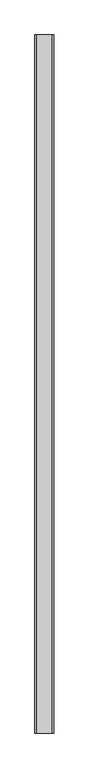
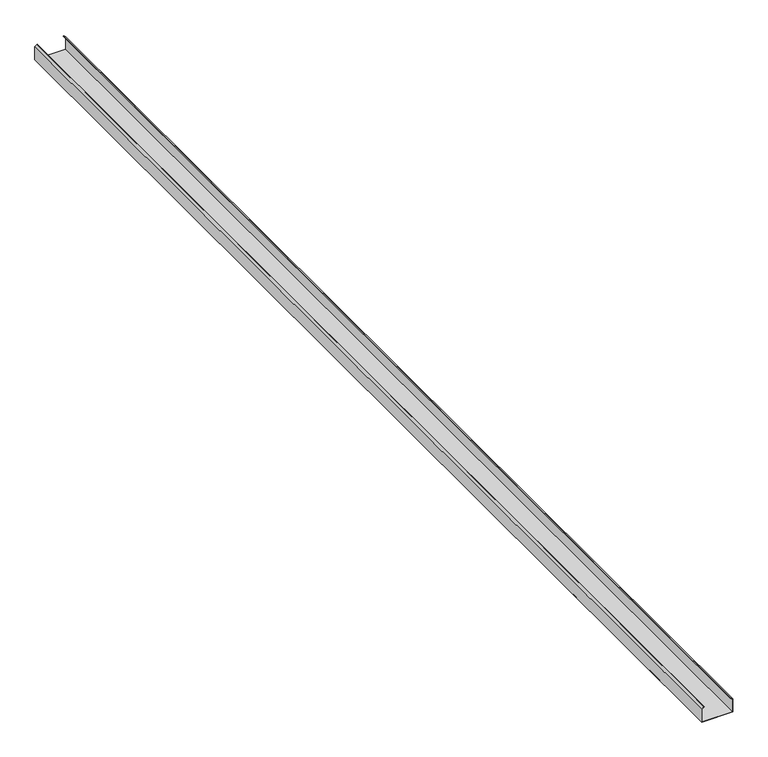
"""IFC4 building model written with IfcOpenShell, lengths in millimetres: proxy geometry, Generic Models 7:Generic Models 1:1:Generic Models 1:1 : Generic Models 7:Generic Models 1:337419:30 : Generic Models 7:Generic Models 1:1:Generic Models 1:1 : Generic Models 7:Generic Models 1:337419:306201."""

from ifc_helpers import new_model, si_unit, frame, origin, place, context, project, spatial, polyline, outline, extrude, source, transform, mapped, element, save


def generic_models_a6c114fe(model_context):
    return source(origin(), model_context, "Body", "SweptSolid", [
        extrude(outline(polyline([(2446.5359375, 667293.3117239), (2446.5359375, 667496.5117239), (2535.4359375, 667496.5117239), (2547.6810414, 667481.9185773), (2545.5528742, 667480.132833), (2534.1404765, 667493.7335989), (2449.3140625, 667493.7335989), (2449.3140625, 667296.0898489), (2534.1404765, 667296.0898489), (2545.5528742, 667309.6906149), (2547.6810414, 667307.9048706), (2535.4359375, 667293.3117239), (2446.5359375, 667293.3117239)])), frame((0.0, -507687.0163841, 0.0), z_axis=(0.0, 1.0, 0.0), x_axis=(0.0, 0.0, 1.0)), (0.0, 0.0, 1.0), 7569.2),
    ])


if __name__ == "__main__":
    model = new_model("IFC4")
    model_context = context("Model", 3, world=origin())
    ifc_project = project(units=[si_unit("LENGTHUNIT", "METRE", prefix="MILLI")], contexts=[model_context])
    site = spatial("IfcSite", under=ifc_project)
    building = spatial("IfcBuilding", under=site)
    placement = place(None, origin())
    generic_models_shape = generic_models_a6c114fe(model_context)
    element("IfcBuildingElementProxy", 1, Name="Generic Models 7:Generic Models 1:1:Generic Models 1:1 : Generic Models 7:Generic Models 1:337419:30 : Generic Models 7:Generic Models 1:1:Generic Models 1:1 : Generic Models 7:Generic Models 1:337419:306201", ObjectType="Generic Models 7:Generic Models 1:1:Generic Models 1:1 : Generic Models 7:Generic Models 1:337419:30 : Generic Models 7:Generic Models 1:1:Generic Models 1:1 : Generic Models 7:Generic Models 1:337419:306201", at=placement, inside=building, context=model_context, shape_type="MappedRepresentation", body=[
        mapped(generic_models_shape, transform((0.0, 0.0, 0.0), x_axis=(1.0, 0.0, 0.0), y_axis=(0.0, 1.0, 0.0), z_axis=(0.0, 0.0, 1.0))),
    ])
    save(model, "model.ifc")

# Revit data of these elements
# Type "Generic Models 7:Generic Models 1:1:Generic Models 1:1 : Generic Models 7:Generic Models 1:337419:30 : Generic Models 7:Generic Models 1:1:Generic Models 1:1 : Generic Models 7:Generic Models 1:337419:306201"
#   NameOverride = "Generic Models 7:Generic Models 1:1:Generic Models 1:1 : Generic Models 7:Generic Models 1:337419:306201"
#   ObjectTypeOverride = "Generic Models 1:1 : Generic Models 7:Generic Models 1:337419"
#   Reference = "Generic Models 1"
#   Tag = "306201"
# Element 1 (IfcBuildingElementProxy, "Generic Models 7:Generic Models 1:1:Generic Models 1:1 : Generic Models 7:Generic Models 1:337419:30 : Generic Models 7:Generic Models 1:1:Generic Models 1:1 : Generic Models 7:Generic Models 1:337419:306201")
#   Materials on its faces: "CEE' SECTION (8.0x3.5C - SEE STRUCT. DWGS)"
# Materials
#   "CEE' SECTION (8.0x3.5C - SEE STRUCT. DWGS)": class "Unassigned", colour RGB 210 209 208, transparency 0, Keynote = "M05121300.02", Cost = 0
